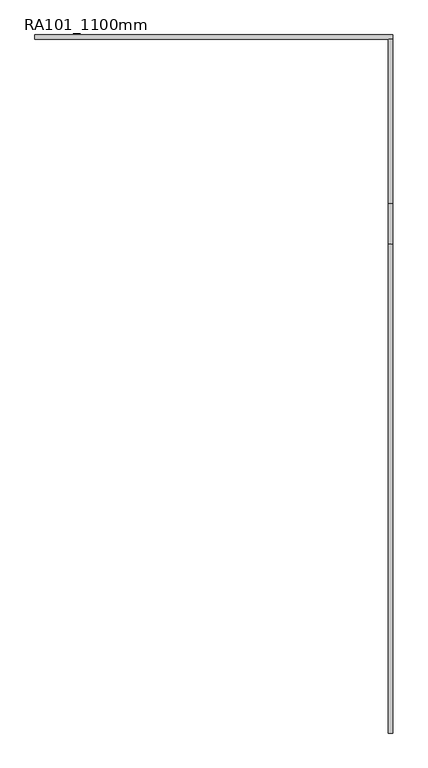
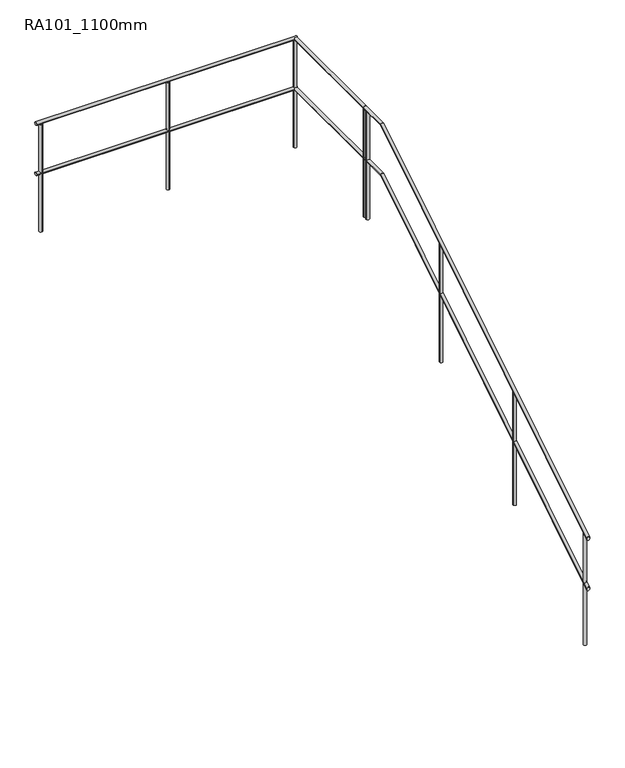
"""IFC4 building model written with IfcOpenShell, lengths in millimetres: railing geometry, RA101_1100mm."""

from ifc_helpers import new_model, si_unit, point, frame, frame_2d, origin, place, context, project, spatial, circle_curve, ellipse_curve, trimmed, segment, composite_curve, outline, extrude, source, transform, mapped, element, save
from ifc_brep_helpers import plane_surface, cylinder_surface, advanced_brep


def ra101_1100mm_f57b0715(model_context):
    return source(origin(), model_context, "Body", "SolidModel", [
        advanced_brep(
        [(12685.1052251, 14699.5208589, 456.3396197), (12655.1052251, 14699.5208589, 456.3396197), (12685.1052251, 18339.5208589, 2547.0), (12655.1052251, 18339.5208589, 2547.0), (12685.1052251, 18063.8019306, 2547.0), (12655.1052251, 18063.8019306, 2547.0)],
        [
            (0, 1, ellipse_curve(frame((12670.1052251, 14699.5208589, 456.3396197), z_axis=(0.0, -1.0, 0.0), x_axis=(0.0, 0.0, -1.0)), 17.6603803, 15.0)),
            (1, 0, ellipse_curve(frame((12670.1052251, 14699.5208589, 456.3396197), z_axis=(0.0, -1.0, 0.0), x_axis=(0.0, 0.0, -1.0)), 17.6603803, 15.0)),
            (2, 3, circle_curve(frame((12670.1052251, 18339.5208589, 2547.0), z_axis=(0.0, 1.0, 0.0), x_axis=(-1.0, 0.0, 0.0)), 15.0)),
            (3, 2, circle_curve(frame((12670.1052251, 18339.5208589, 2547.0), z_axis=(0.0, 1.0, 0.0), x_axis=(-1.0, 0.0, 0.0)), 15.0)),
            (0, 4),
            (4, 5, ellipse_curve(frame((12670.1052251, 18063.8019306, 2547.0), z_axis=(0.0, -0.9616025257983003, -0.2744459552959912), x_axis=(0.0, 0.2744459552959914, -0.9616025257983002)), 15.5989607, 15.0)),
            (5, 1),
            (5, 4, ellipse_curve(frame((12670.1052251, 18063.8019306, 2547.0), z_axis=(0.0, -0.9616025257983003, -0.2744459552959912), x_axis=(0.0, 0.2744459552959914, -0.9616025257983002)), 15.5989607, 15.0)),
            (4, 2),
            (3, 5),
        ],
        [
            plane_surface(frame((12670.1052251, 14699.5208589, 474.0), z_axis=(0.0, -1.0, 0.0), x_axis=(0.0, 0.0, 1.0))),
            plane_surface(frame((12670.1052251, 18339.5208589, 2562.0), z_axis=(0.0, 1.0, 0.0), x_axis=(0.0, 0.0, 1.0))),
            cylinder_surface(frame((12670.1052251, 14707.4380966, 461.2596175), z_axis=(0.0, -0.8493588352433417, -0.5278158476155052), x_axis=(-1.0, 0.0, 0.0)), 15.0),
            cylinder_surface(frame((12670.1052251, 18059.5208589, 2547.0), z_axis=(0.0, -1.0, 0.0), x_axis=(-1.0, 0.0, 0.0)), 15.0),
        ],
        [
            (0, [[1, 2]]),
            (1, [[3, 4]]),
            (2, [[-1, 5, 6, 7]]),
            (2, [[-2, -7, 8, -5]]),
            (3, [[-6, 9, -4, 10]]),
            (3, [[-8, -10, -3, -9]]),
        ],
    ),
        advanced_brep(
        [(12685.1052251, 18339.5208589, 2547.0), (12655.1052251, 18339.5208589, 2547.0), (12685.1052251, 19469.5208589, 2547.0), (12655.1052251, 19469.5208589, 2547.0)],
        [
            (0, 1, circle_curve(frame((12670.1052251, 18339.5208589, 2547.0), z_axis=(0.0, -1.0, 0.0), x_axis=(-1.0, 0.0, 0.0)), 15.0)),
            (1, 0, circle_curve(frame((12670.1052251, 18339.5208589, 2547.0), z_axis=(0.0, -1.0, 0.0), x_axis=(-1.0, 0.0, 0.0)), 15.0)),
            (2, 3, circle_curve(frame((12670.1052251, 19469.5208589, 2547.0), z_axis=(0.0, 1.0, 0.0), x_axis=(-1.0, 0.0, 0.0)), 15.0)),
            (3, 2, circle_curve(frame((12670.1052251, 19469.5208589, 2547.0), z_axis=(0.0, 1.0, 0.0), x_axis=(-1.0, 0.0, 0.0)), 15.0)),
            (0, 2),
            (3, 1),
        ],
        [
            plane_surface(frame((12670.1052251, 18339.5208589, 2562.0), z_axis=(0.0, -1.0, 0.0), x_axis=(0.0, 0.0, 1.0))),
            plane_surface(frame((12670.1052251, 19469.5208589, 2562.0), z_axis=(0.0, 1.0, 0.0), x_axis=(0.0, 0.0, 1.0))),
            cylinder_surface(frame((12670.1052251, 18339.5208589, 2547.0), z_axis=(0.0, -1.0, 0.0), x_axis=(-1.0, 0.0, 0.0)), 15.0),
        ],
        [
            (0, [[1, 2]]),
            (1, [[3, 4]]),
            (2, [[-1, 5, -4, 6]]),
            (2, [[-2, -6, -3, -5]]),
        ],
    ),
        advanced_brep(
        [(12685.1052251, 19499.5208589, 2547.0), (12685.1052251, 19469.5208589, 2547.0), (10225.1052251, 19499.5208589, 2547.0), (10225.1052251, 19469.5208589, 2547.0)],
        [
            (0, 1, circle_curve(frame((12685.1052251, 19484.5208589, 2547.0), z_axis=(1.0, 0.0, 0.0), x_axis=(0.0, -1.0, 0.0)), 15.0)),
            (1, 0, circle_curve(frame((12685.1052251, 19484.5208589, 2547.0), z_axis=(1.0, 0.0, 0.0), x_axis=(0.0, -1.0, 0.0)), 15.0)),
            (2, 3, circle_curve(frame((10225.1052251, 19484.5208589, 2547.0), z_axis=(-1.0, 0.0, 0.0), x_axis=(0.0, -1.0, 0.0)), 15.0)),
            (3, 2, circle_curve(frame((10225.1052251, 19484.5208589, 2547.0), z_axis=(-1.0, 0.0, 0.0), x_axis=(0.0, -1.0, 0.0)), 15.0)),
            (0, 2),
            (3, 1),
        ],
        [
            plane_surface(frame((12685.1052251, 19484.5208589, 2562.0), z_axis=(1.0, 0.0, 0.0), x_axis=(0.0, -1.0, 0.0))),
            plane_surface(frame((10225.1052251, 19484.5208589, 2562.0), z_axis=(-1.0, 0.0, 0.0), x_axis=(0.0, -1.0, 0.0))),
            cylinder_surface(frame((12685.1052251, 19484.5208589, 2547.0), z_axis=(1.0, 0.0, 0.0), x_axis=(0.0, -1.0, 0.0)), 15.0),
        ],
        [
            (0, [[1, 2]]),
            (1, [[3, 4]]),
            (2, [[-1, 5, -4, 6]]),
            (2, [[-2, -6, -3, -5]]),
        ],
    ),
        advanced_brep(
        [(12685.1052251, 14699.5208589, 956.3396197), (12655.1052251, 14699.5208589, 956.3396197), (12685.1052251, 18063.8019306, 3047.0), (12655.1052251, 18063.8019306, 3047.0), (12685.1052251, 18339.5208589, 3047.0), (12655.1052251, 18339.5208589, 3047.0)],
        [
            (0, 1, ellipse_curve(frame((12670.1052251, 14699.5208589, 956.3396197), z_axis=(0.0, -1.0, 0.0), x_axis=(0.0, 0.0, -1.0)), 17.6603803, 15.0)),
            (1, 0, ellipse_curve(frame((12670.1052251, 14699.5208589, 956.3396197), z_axis=(0.0, -1.0, 0.0), x_axis=(0.0, 0.0, -1.0)), 17.6603803, 15.0)),
            (0, 2),
            (2, 3, ellipse_curve(frame((12670.1052251, 18063.8019306, 3047.0), z_axis=(0.0, -0.9616025257983003, -0.2744459552959912), x_axis=(0.0, 0.2744459552959914, -0.9616025257983002)), 15.5989607, 15.0)),
            (3, 1),
            (3, 2, ellipse_curve(frame((12670.1052251, 18063.8019306, 3047.0), z_axis=(0.0, -0.9616025257983003, -0.2744459552959912), x_axis=(0.0, 0.2744459552959914, -0.9616025257983002)), 15.5989607, 15.0)),
            (4, 5, circle_curve(frame((12670.1052251, 18339.5208589, 3047.0), z_axis=(0.0, 1.0, 0.0), x_axis=(-1.0, 0.0, 0.0)), 15.0)),
            (5, 4, circle_curve(frame((12670.1052251, 18339.5208589, 3047.0), z_axis=(0.0, 1.0, 0.0), x_axis=(-1.0, 0.0, 0.0)), 15.0)),
            (2, 4),
            (5, 3),
        ],
        [
            plane_surface(frame((12670.1052251, 14699.5208589, 974.0), z_axis=(0.0, -1.0, 0.0), x_axis=(0.0, 0.0, 1.0))),
            cylinder_surface(frame((12670.1052251, 14707.4380966, 961.2596175), z_axis=(0.0, -0.8493588352433417, -0.5278158476155052), x_axis=(-1.0, 0.0, 0.0)), 15.0),
            plane_surface(frame((12670.1052251, 18339.5208589, 3062.0), z_axis=(0.0, 1.0, 0.0), x_axis=(0.0, 0.0, 1.0))),
            cylinder_surface(frame((12670.1052251, 18059.5208589, 3047.0), z_axis=(0.0, -1.0, 0.0), x_axis=(-1.0, 0.0, 0.0)), 15.0),
        ],
        [
            (0, [[1, 2]]),
            (1, [[-1, 3, 4, 5]]),
            (1, [[-2, -5, 6, -3]]),
            (2, [[7, 8]]),
            (3, [[-4, 9, -8, 10]]),
            (3, [[-6, -10, -7, -9]]),
        ],
    ),
        advanced_brep(
        [(12685.1052251, 18339.5208589, 3047.0), (12655.1052251, 18339.5208589, 3047.0), (12685.1052251, 19469.5208589, 3047.0), (12655.1052251, 19469.5208589, 3047.0)],
        [
            (0, 1, circle_curve(frame((12670.1052251, 18339.5208589, 3047.0), z_axis=(0.0, -1.0, 0.0), x_axis=(-1.0, 0.0, 0.0)), 15.0)),
            (1, 0, circle_curve(frame((12670.1052251, 18339.5208589, 3047.0), z_axis=(0.0, -1.0, 0.0), x_axis=(-1.0, 0.0, 0.0)), 15.0)),
            (2, 3, circle_curve(frame((12670.1052251, 19469.5208589, 3047.0), z_axis=(0.0, 1.0, 0.0), x_axis=(-1.0, 0.0, 0.0)), 15.0)),
            (3, 2, circle_curve(frame((12670.1052251, 19469.5208589, 3047.0), z_axis=(0.0, 1.0, 0.0), x_axis=(-1.0, 0.0, 0.0)), 15.0)),
            (0, 2),
            (3, 1),
        ],
        [
            plane_surface(frame((12670.1052251, 18339.5208589, 3062.0), z_axis=(0.0, -1.0, 0.0), x_axis=(0.0, 0.0, 1.0))),
            plane_surface(frame((12670.1052251, 19469.5208589, 3062.0), z_axis=(0.0, 1.0, 0.0), x_axis=(0.0, 0.0, 1.0))),
            cylinder_surface(frame((12670.1052251, 18339.5208589, 3047.0), z_axis=(0.0, -1.0, 0.0), x_axis=(-1.0, 0.0, 0.0)), 15.0),
        ],
        [
            (0, [[1, 2]]),
            (1, [[3, 4]]),
            (2, [[-1, 5, -4, 6]]),
            (2, [[-2, -6, -3, -5]]),
        ],
    ),
        advanced_brep(
        [(12685.1052251, 19499.5208589, 3047.0), (12685.1052251, 19469.5208589, 3047.0), (10225.1052251, 19499.5208589, 3047.0), (10225.1052251, 19469.5208589, 3047.0)],
        [
            (0, 1, circle_curve(frame((12685.1052251, 19484.5208589, 3047.0), z_axis=(1.0, 0.0, 0.0), x_axis=(0.0, -1.0, 0.0)), 15.0)),
            (1, 0, circle_curve(frame((12685.1052251, 19484.5208589, 3047.0), z_axis=(1.0, 0.0, 0.0), x_axis=(0.0, -1.0, 0.0)), 15.0)),
            (2, 3, circle_curve(frame((10225.1052251, 19484.5208589, 3047.0), z_axis=(-1.0, 0.0, 0.0), x_axis=(0.0, -1.0, 0.0)), 15.0)),
            (3, 2, circle_curve(frame((10225.1052251, 19484.5208589, 3047.0), z_axis=(-1.0, 0.0, 0.0), x_axis=(0.0, -1.0, 0.0)), 15.0)),
            (0, 2),
            (3, 1),
        ],
        [
            plane_surface(frame((12685.1052251, 19484.5208589, 3062.0), z_axis=(1.0, 0.0, 0.0), x_axis=(0.0, -1.0, 0.0))),
            plane_surface(frame((10225.1052251, 19484.5208589, 3062.0), z_axis=(-1.0, 0.0, 0.0), x_axis=(0.0, -1.0, 0.0))),
            cylinder_surface(frame((12685.1052251, 19484.5208589, 3047.0), z_axis=(1.0, 0.0, 0.0), x_axis=(0.0, -1.0, 0.0)), 15.0),
        ],
        [
            (0, [[1, 2]]),
            (1, [[3, 4]]),
            (2, [[-1, 5, -4, 6]]),
            (2, [[-2, -6, -3, -5]]),
        ],
    ),
        extrude(outline(composite_curve([segment(trimmed(circle_curve(frame_2d((10270.1052251, 19484.5208589)), 15.0), [point((10270.1052251, 19469.5208589))], [point((10270.1052251, 19499.5208589))], False, "CARTESIAN"), True, "CONTINUOUS"), segment(trimmed(circle_curve(frame_2d((10270.1052251, 19484.5208589)), 15.0), [point((10270.1052251, 19499.5208589))], [point((10270.1052251, 19469.5208589))], False, "CARTESIAN"), True, "CONTINUOUS")], self_intersect=False)), frame((0.0, 0.0, 1962.0), z_axis=(0.0, 0.0, 1.0), x_axis=(1.0, 0.0, 0.0)), (0.0, 0.0, 1.0), 1070.0),
        extrude(outline(composite_curve([segment(trimmed(circle_curve(frame_2d((11470.1052251, 19484.5208589)), 15.0), [point((11470.1052251, 19469.5208589))], [point((11470.1052251, 19499.5208589))], False, "CARTESIAN"), True, "CONTINUOUS"), segment(trimmed(circle_curve(frame_2d((11470.1052251, 19484.5208589)), 15.0), [point((11470.1052251, 19499.5208589))], [point((11470.1052251, 19469.5208589))], False, "CARTESIAN"), True, "CONTINUOUS")], self_intersect=False)), frame((0.0, 0.0, 1962.0), z_axis=(0.0, 0.0, 1.0), x_axis=(1.0, 0.0, 0.0)), (0.0, 0.0, 1.0), 1070.0),
        extrude(outline(composite_curve([segment(trimmed(circle_curve(frame_2d((12670.1052251, 18299.5208589)), 15.0), [point((12655.1052251, 18299.5208589))], [point((12685.1052251, 18299.5208589))], False, "CARTESIAN"), True, "CONTINUOUS"), segment(trimmed(circle_curve(frame_2d((12670.1052251, 18299.5208589)), 15.0), [point((12685.1052251, 18299.5208589))], [point((12655.1052251, 18299.5208589))], False, "CARTESIAN"), True, "CONTINUOUS")], self_intersect=False)), frame((0.0, 0.0, 1962.0), z_axis=(0.0, 0.0, 1.0), x_axis=(1.0, 0.0, 0.0)), (0.0, 0.0, 1.0), 1070.0),
        extrude(outline(composite_curve([segment(trimmed(circle_curve(frame_2d((12670.1052251, 17099.5208589)), 15.0), [point((12655.1052251, 17099.5208589))], [point((12685.1052251, 17099.5208589))], False, "CARTESIAN"), True, "CONTINUOUS"), segment(trimmed(circle_curve(frame_2d((12670.1052251, 17099.5208589)), 15.0), [point((12685.1052251, 17099.5208589))], [point((12655.1052251, 17099.5208589))], False, "CARTESIAN"), True, "CONTINUOUS")], self_intersect=False)), frame((0.0, 0.0, 1266.0), z_axis=(0.0, 0.0, 1.0), x_axis=(1.0, 0.0, 0.0)), (0.0, 0.0, 1.0), 1169.4285714),
        extrude(outline(composite_curve([segment(trimmed(circle_curve(frame_2d((12670.1052251, 15899.5208589)), 15.0), [point((12655.1052251, 15899.5208589))], [point((12685.1052251, 15899.5208589))], False, "CARTESIAN"), True, "CONTINUOUS"), segment(trimmed(circle_curve(frame_2d((12670.1052251, 15899.5208589)), 15.0), [point((12685.1052251, 15899.5208589))], [point((12655.1052251, 15899.5208589))], False, "CARTESIAN"), True, "CONTINUOUS")], self_intersect=False)), frame((0.0, 0.0, 570.0), z_axis=(0.0, 0.0, 1.0), x_axis=(1.0, 0.0, 0.0)), (0.0, 0.0, 1.0), 1119.7142857),
        extrude(outline(composite_curve([segment(trimmed(circle_curve(frame_2d((12670.1052251, 19484.5208589)), 15.0), [point((12655.1052251, 19484.5208589))], [point((12685.1052251, 19484.5208589))], False, "CARTESIAN"), True, "CONTINUOUS"), segment(trimmed(circle_curve(frame_2d((12670.1052251, 19484.5208589)), 15.0), [point((12685.1052251, 19484.5208589))], [point((12655.1052251, 19484.5208589))], False, "CARTESIAN"), True, "CONTINUOUS")], self_intersect=False)), frame((0.0, 0.0, 1962.0), z_axis=(0.0, 0.0, 1.0), x_axis=(1.0, 0.0, 0.0)), (0.0, 0.0, 1.0), 1070.0),
        extrude(outline(composite_curve([segment(trimmed(circle_curve(frame_2d((12670.1052251, 18339.5208589)), 15.0), [point((12655.1052251, 18339.5208589))], [point((12685.1052251, 18339.5208589))], False, "CARTESIAN"), True, "CONTINUOUS"), segment(trimmed(circle_curve(frame_2d((12670.1052251, 18339.5208589)), 15.0), [point((12685.1052251, 18339.5208589))], [point((12655.1052251, 18339.5208589))], False, "CARTESIAN"), True, "CONTINUOUS")], self_intersect=False)), frame((0.0, 0.0, 1962.0), z_axis=(0.0, 0.0, 1.0), x_axis=(1.0, 0.0, 0.0)), (0.0, 0.0, 1.0), 1070.0),
        extrude(outline(composite_curve([segment(trimmed(circle_curve(frame_2d((10275.1052251, 19484.5208589)), 15.0), [point((10275.1052251, 19469.5208589))], [point((10275.1052251, 19499.5208589))], False, "CARTESIAN"), True, "CONTINUOUS"), segment(trimmed(circle_curve(frame_2d((10275.1052251, 19484.5208589)), 15.0), [point((10275.1052251, 19499.5208589))], [point((10275.1052251, 19469.5208589))], False, "CARTESIAN"), True, "CONTINUOUS")], self_intersect=False)), frame((0.0, 0.0, 1962.0), z_axis=(0.0, 0.0, 1.0), x_axis=(1.0, 0.0, 0.0)), (0.0, 0.0, 1.0), 1070.0),
        extrude(outline(composite_curve([segment(trimmed(circle_curve(frame_2d((12670.1052251, 14749.5208589)), 15.0), [point((12655.1052251, 14749.5208589))], [point((12685.1052251, 14749.5208589))], False, "CARTESIAN"), True, "CONTINUOUS"), segment(trimmed(circle_curve(frame_2d((12670.1052251, 14749.5208589)), 15.0), [point((12685.1052251, 14749.5208589))], [point((12655.1052251, 14749.5208589))], False, "CARTESIAN"), True, "CONTINUOUS")], self_intersect=False)), frame((0.0, 0.0, -126.0), z_axis=(0.0, 0.0, 1.0), x_axis=(1.0, 0.0, 0.0)), (0.0, 0.0, 1.0), 1101.0714286),
    ])


if __name__ == "__main__":
    model = new_model("IFC4")
    model_context = context("Model", 3, world=origin())
    ifc_project = project(units=[si_unit("LENGTHUNIT", "METRE", prefix="MILLI")], contexts=[model_context])
    site = spatial("IfcSite", under=ifc_project)
    building = spatial("IfcBuilding", under=site)
    placement = place(None, origin())
    ra101_1100mm_shape = ra101_1100mm_f57b0715(model_context)
    element("IfcRailing", 1, ObjectType="RA101_1100mm", at=placement, inside=building, context=model_context, shape_type="MappedRepresentation", body=[
        mapped(ra101_1100mm_shape, transform((0.0, 0.0, 0.0), x_axis=(1.0, 0.0, 0.0), y_axis=(0.0, 1.0, 0.0), z_axis=(0.0, 0.0, 1.0))),
    ])
    save(model, "model.ifc")
